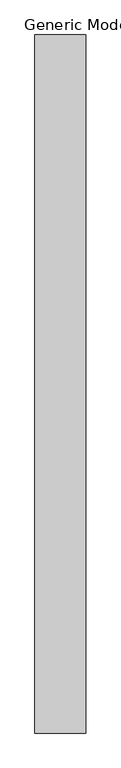
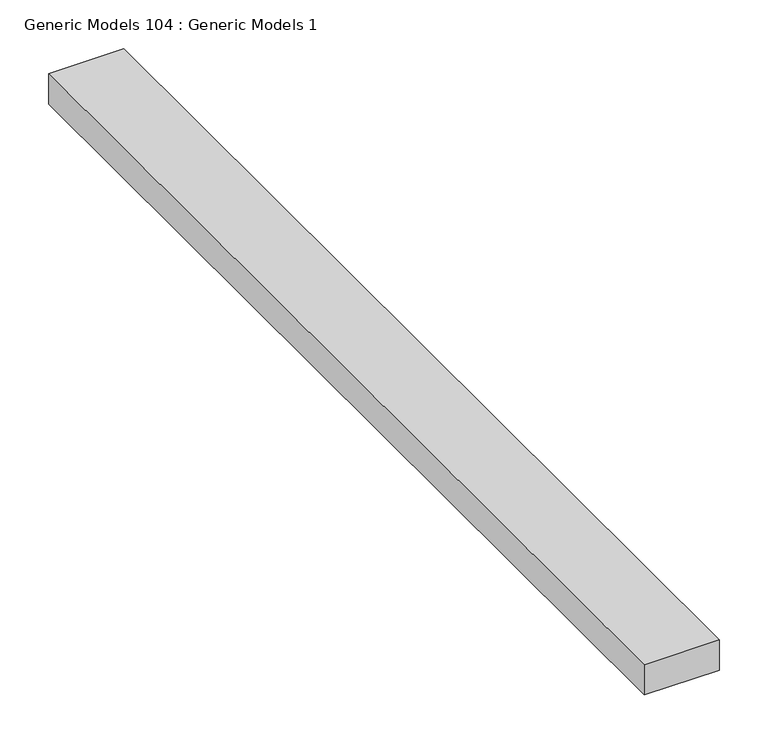
"""IFC4 building model written with IfcOpenShell, lengths in millimetres: proxy geometry, Generic Models 104 : Generic Models 1."""

from ifc_helpers import new_model, si_unit, frame, origin, place, context, project, spatial, polyline, outline, extrude, source, transform, mapped, element, save


def generic_models_104_generic_models_1_af33e5d9(model_context):
    return source(origin(), model_context, "Body", "SweptSolid", [
        extrude(outline(polyline([(52206.021109, 0.0), (52117.121109, 0.0), (52117.121109, 1219.2), (52206.021109, 1219.2), (52206.021109, 0.0)])), frame((0.0, 0.0, 4412.45625), z_axis=(0.0, 0.0, 1.0), x_axis=(1.0, 0.0, 0.0)), (0.0, 0.0, 1.0), 38.1),
    ])


if __name__ == "__main__":
    model = new_model("IFC4")
    model_context = context("Model", 3, world=origin())
    ifc_project = project(units=[si_unit("LENGTHUNIT", "METRE", prefix="MILLI")], contexts=[model_context])
    site = spatial("IfcSite", under=ifc_project)
    building = spatial("IfcBuilding", under=site)
    placement = place(None, origin())
    generic_models_104_generic_models_1_shape = generic_models_104_generic_models_1_af33e5d9(model_context)
    element("IfcBuildingElementProxy", 1, Name="Generic Models 104 : Generic Models 1", ObjectType="Generic Models 104 : Generic Models 1", at=placement, inside=building, context=model_context, shape_type="MappedRepresentation", body=[
        mapped(generic_models_104_generic_models_1_shape, transform((0.0, 0.0, 0.0), x_axis=(1.0, 0.0, 0.0), y_axis=(0.0, 1.0, 0.0), z_axis=(0.0, 0.0, 1.0))),
    ])
    save(model, "model.ifc")

# Revit data of these elements
# Element 1 (IfcBuildingElementProxy, "Generic Models 104 : Generic Models 1")
#   Materials on its faces: "WOOD BLOCKING - SIZE AS NECESSARY"
# Materials
#   "WOOD BLOCKING - SIZE AS NECESSARY": class "Wood", colour RGB 234 198 147, transparency 0, Description = "Pinus Echinata", Cost = 0
